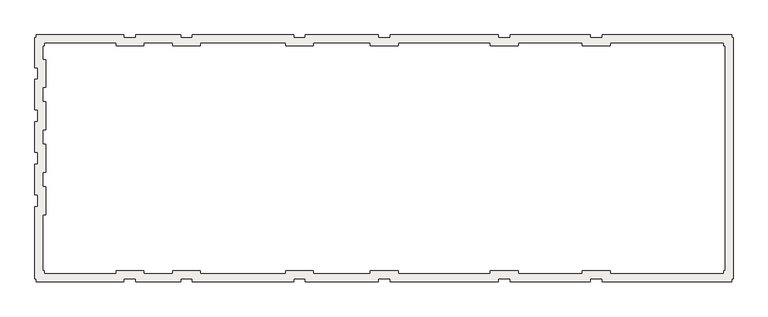
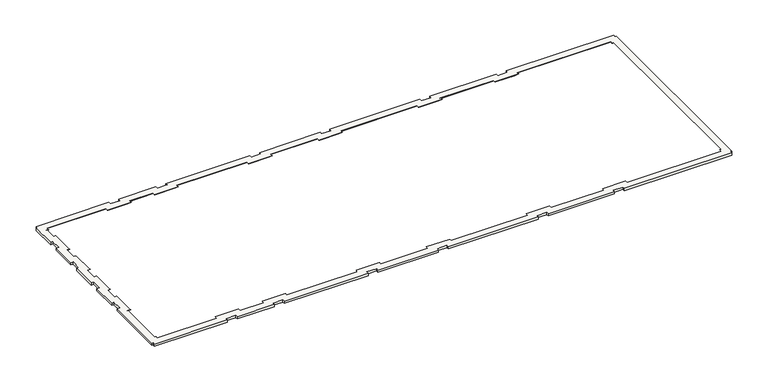
"""IFC4 building model written with IfcOpenShell, lengths in millimetres: slab geometry, HAUNCH FOR SOG : FTS801_Haunch_GS."""

import ifcopenshell
import ifcopenshell.guid

model = None  # the IFC model being written
_history = None  # IfcOwnerHistory: only IFC2X3 demands one
_inside = {}  # id of a spatial element -> (the spatial element, [elements in it])
_under = {}  # id of a project, library or spatial element -> (it, [spatial elements below it])
_declared = {}  # id of a project -> (the project, [libraries it declares])
_typed = {}  # id of a type object -> (the type object, [elements of that type])
_made_of = {}  # id of a material, layer set ... -> (it, [elements and type objects made of it])


def new_model(schema):
    """Start an empty IFC model of exactly this schema.

    Asked for "IFC4X3", IfcOpenShell would pick the latest addendum, in which some entities
    have other attributes; the version numbers below select the first issue.
    IFC2X3 requires an IfcOwnerHistory on every rooted entity: one is made here for all.
    """
    global model, _history
    if schema == "IFC4X3":
        model = ifcopenshell.file(schema_version=(4, 3, 0, 0))
    else:
        model = ifcopenshell.file(schema=schema)
    _inside.clear()
    _under.clear()
    _declared.clear()
    _typed.clear()
    _made_of.clear()
    _history = None
    if model.schema == "IFC2X3":
        org = make("IfcOrganization", Name="unknown")
        user = make(
            "IfcPersonAndOrganization",
            ThePerson=make("IfcPerson", FamilyName="unknown"),
            TheOrganization=org,
        )
        app = make(
            "IfcApplication",
            ApplicationDeveloper=org,
            Version="unknown",
            ApplicationFullName="unknown",
            ApplicationIdentifier="unknown",
        )
        _history = make(
            "IfcOwnerHistory",
            OwningUser=user,
            OwningApplication=app,
            ChangeAction="ADDED",
            CreationDate=0,
        )
    return model


def make(cls, **values):
    """One entity of the class cls with the attributes given. An attribute that is None is left unset."""
    return model.create_entity(
        cls, **{name: value for name, value in values.items() if value is not None}
    )


def rooted(cls, **values):
    """An entity with a GlobalId (a new one), such as an element, a storey or a relation."""
    return make(cls, GlobalId=ifcopenshell.guid.new(), OwnerHistory=_history, **values)


def si_unit(unit_type, name, prefix=None):
    """IfcSIUnit, for example si_unit("LENGTHUNIT", "METRE", prefix="MILLI")."""
    return make("IfcSIUnit", UnitType=unit_type, Prefix=prefix, Name=name)


def assignment(units):
    """IfcUnitAssignment: the units of a project."""
    return None if units is None else make("IfcUnitAssignment", Units=units)


def point(xyz):
    """IfcCartesianPoint."""
    return None if xyz is None else make("IfcCartesianPoint", Coordinates=xyz)


def direction(xyz):
    """IfcDirection."""
    return None if xyz is None else make("IfcDirection", DirectionRatios=xyz)


def frame(location, z_axis=None, x_axis=None):
    """IfcAxis2Placement3D, a coordinate frame: its origin and axes. An axis left out is left unset."""
    return make(
        "IfcAxis2Placement3D",
        Location=point(location),
        Axis=direction(z_axis),
        RefDirection=direction(x_axis),
    )


def origin():
    """The frame at (0, 0, 0) with its axes left unset."""
    return frame((0.0, 0.0, 0.0))


def place(relative_to, where):
    """IfcLocalPlacement: puts the frame where relative to a parent placement (None: the world)."""
    return make(
        "IfcLocalPlacement", PlacementRelTo=relative_to, RelativePlacement=where
    )


def context(
    kind, dimensions, precision=None, world=None, true_north=None, identifier=None
):
    """IfcGeometricRepresentationContext, for example the 3D "Model" context."""
    return make(
        "IfcGeometricRepresentationContext",
        ContextIdentifier=identifier,
        ContextType=kind,
        CoordinateSpaceDimension=dimensions,
        Precision=precision,
        WorldCoordinateSystem=world,
        TrueNorth=true_north,
    )


def project(units=None, contexts=None):
    """IfcProject with its units and contexts."""
    return rooted(
        "IfcProject",
        Name="project",
        RepresentationContexts=contexts,
        UnitsInContext=assignment(units),
    )


def spatial(cls, under=None, at=None, **own):
    """A site, building, storey or space (cls), placed at a placement, below another one or the project."""
    s = rooted(cls, ObjectPlacement=at, **own)
    if under is not None:
        _under.setdefault(under.id(), (under, []))[1].append(s)
    return s


def faces_of(points, faces, orient=None, outer=None):
    """IfcFace entities. A face is a list of loops; a loop is a list of indices into points, from 0.

    orient and outer hold one flag for each loop. By default every Orientation is true, the
    first loop of a face is its IfcFaceOuterBound and the others are IfcFaceBound.
    """
    made = []
    for i, loops in enumerate(faces):
        bounds = []
        for j, loop in enumerate(loops):
            is_outer = j == 0 if outer is None else outer[i][j]
            bounds.append(
                make(
                    "IfcFaceOuterBound" if is_outer else "IfcFaceBound",
                    Bound=make("IfcPolyLoop", Polygon=[points[k] for k in loop]),
                    Orientation=True if orient is None else orient[i][j],
                )
            )
        made.append(make("IfcFace", Bounds=bounds))
    return made


def faceted_brep(points, faces, orient=None, outer=None, voids=None):
    """IfcFacetedBrep: a solid bounded by flat faces; with voids (closed shells), ...WithVoids."""
    shared = [point(p) for p in points]
    hull = make("IfcClosedShell", CfsFaces=faces_of(shared, faces, orient, outer))
    if voids is None:
        return make("IfcFacetedBrep", Outer=hull)
    return make(
        "IfcFacetedBrepWithVoids",
        Outer=hull,
        Voids=[
            make(cls, CfsFaces=faces_of(shared, fs, o, b)) for cls, fs, o, b in voids
        ],
    )


def shape(context_of_items, identifier, shape_type, items):
    """IfcShapeRepresentation: the items that make up one representation, for example the "Body"."""
    return make(
        "IfcShapeRepresentation",
        ContextOfItems=context_of_items,
        RepresentationIdentifier=identifier,
        RepresentationType=shape_type,
        Items=items,
    )


def source(mapping_origin, context_of_items, identifier, shape_type, items):
    """IfcRepresentationMap: a shape defined once, which mapped items show again and again."""
    return make(
        "IfcRepresentationMap",
        MappingOrigin=mapping_origin,
        MappedRepresentation=shape(context_of_items, identifier, shape_type, items),
    )


def transform(
    local_origin,
    x_axis=None,
    y_axis=None,
    z_axis=None,
    scale=None,
    scale2=None,
    scale3=None,
    uniform=True,
):
    """IfcCartesianTransformationOperator3D, or its non-uniform kind. x_axis, y_axis, z_axis: its Axis1, 2, 3."""
    if uniform:
        return make(
            "IfcCartesianTransformationOperator3D",
            Axis1=direction(x_axis),
            Axis2=direction(y_axis),
            LocalOrigin=point(local_origin),
            Scale=scale,
            Axis3=direction(z_axis),
        )
    return make(
        "IfcCartesianTransformationOperator3DnonUniform",
        Axis1=direction(x_axis),
        Axis2=direction(y_axis),
        LocalOrigin=point(local_origin),
        Scale=scale,
        Axis3=direction(z_axis),
        Scale2=scale2,
        Scale3=scale3,
    )


def mapped(mapping_source, mapping_target):
    """IfcMappedItem: shows the shape of a source again, moved by a transform."""
    return make(
        "IfcMappedItem", MappingSource=mapping_source, MappingTarget=mapping_target
    )


def made_of(thing, what):
    """Note that an element or type object is made of a material, layer set ...; save() writes the relation."""
    if what is not None:
        _made_of.setdefault(what.id(), (what, []))[1].append(thing)
    return thing


def element(
    cls,
    number,
    at=None,
    inside=None,
    cuts=None,
    type_object=None,
    material=None,
    context=None,
    identifier="Body",
    shape_type=None,
    held_by="IfcProductDefinitionShape",
    body=None,
    shapes=None,
    **own,
):
    """One element of the class cls, such as IfcWall. Its Tag is "e" and its number.

    at: its placement. inside: the storey or other place that contains it. cuts: it is an
    opening in that element (IfcRelVoidsElement). A single representation is given by context,
    identifier, shape_type and body (its items); several are given by shapes. held_by: the class
    of the entity that holds the representations. save() writes the other relations.
    """
    e = rooted(cls, Tag="e%d" % number, ObjectPlacement=at, **own)
    if body is not None:
        shapes = [shape(context, identifier, shape_type, body)]
    if shapes is not None:
        e.Representation = make(held_by, Representations=shapes)
    if inside is not None:
        _inside.setdefault(inside.id(), (inside, []))[1].append(e)
    if cuts is not None:
        rooted(
            "IfcRelVoidsElement", RelatingBuildingElement=cuts, RelatedOpeningElement=e
        )
    if type_object is not None:
        _typed.setdefault(type_object.id(), (type_object, []))[1].append(e)
    return made_of(e, material)


def aggregate(whole, parts):
    """IfcRelAggregates: a whole, such as a stair, and the parts it consists of."""
    return rooted("IfcRelAggregates", RelatingObject=whole, RelatedObjects=parts)


def save(model, path):
    """Write the relations noted so far, then the file.

    IfcRelAggregates (storeys below a building ...), IfcRelContainedInSpatialStructure (elements
    in a storey), IfcRelDefinesByType, IfcRelAssociatesMaterial and IfcRelDeclares: one each for
    every whole, place, type object, material and project.
    """
    for whole, parts in _under.values():
        aggregate(whole, parts)
    for where, things in _inside.values():
        rooted(
            "IfcRelContainedInSpatialStructure",
            RelatedElements=things,
            RelatingStructure=where,
        )
    for kind, things in _typed.values():
        rooted("IfcRelDefinesByType", RelatedObjects=things, RelatingType=kind)
    for what, things in _made_of.values():
        rooted("IfcRelAssociatesMaterial", RelatedObjects=things, RelatingMaterial=what)
    for by, libraries in _declared.values():
        rooted("IfcRelDeclares", RelatingContext=by, RelatedDefinitions=libraries)
    model.write(path)


def slab_ae3d626d(model_context):
    return source(origin(), model_context, "Body", "Brep", [
        faceted_brep([(370.0, 38729.5208589, 399.9720055), (370.0, 38729.5208589, 199.9720055), (370.0, 38529.5208589, 199.9720055), (370.0, 38529.5208589, 399.9720055), (770.0, 38329.5208589, 199.9720055), (970.0, 38129.5208589, 399.9720055), (970.0, 37929.5208589, 399.9720055), (770.0, 38129.5208589, 199.9720055), (270.0, 38529.5208589, 199.9720055), (270.0, 38529.5208589, 399.9720055), (870.0, 37929.5208589, 399.9720055), (670.0, 38129.5208589, 199.9720055), (270.0, 36419.5208589, 199.9720055), (270.0, 36419.5208589, 399.9720055), (870.0, 37019.5208589, 399.9720055), (670.0, 36819.5208589, 199.9720055), (470.0, 36419.5208589, 199.9720055), (470.0, 36419.5208589, 399.9720055), (405.0, 36419.5208589, 399.9720055), (1070.0, 37019.5208589, 399.9720055), (870.0, 36819.5208589, 199.9720055), (470.0, 35579.5208589, 199.9720055), (470.0, 35579.5208589, 399.9720055), (1070.0, 34979.5208589, 399.9720055), (870.0, 35179.5208589, 199.9720055), (270.0, 35579.5208589, 199.9720055), (270.0, 35579.5208589, 399.9720055), (405.0, 35579.5208589, 399.9720055), (870.0, 34979.5208589, 399.9720055), (670.0, 35179.5208589, 199.9720055), (270.0, 33419.5208589, 199.9720055), (270.0, 33419.5208589, 399.9720055), (870.0, 34019.5208589, 399.9720055), (670.0, 33819.5208589, 199.9720055), (470.0, 33419.5208589, 199.9720055), (470.0, 33419.5208589, 399.9720055), (405.0, 33419.5208589, 399.9720055), (1070.0, 34019.5208589, 399.9720055), (870.0, 33819.5208589, 199.9720055), (470.0, 32579.5208589, 199.9720055), (470.0, 32579.5208589, 399.9720055), (1070.0, 31979.5208589, 399.9720055), (870.0, 32179.5208589, 199.9720055), (270.0, 32579.5208589, 199.9720055), (270.0, 32579.5208589, 399.9720055), (405.0, 32579.5208589, 399.9720055), (870.0, 31979.5208589, 399.9720055), (670.0, 32179.5208589, 199.9720055), (270.0, 30419.5208589, 199.9720055), (270.0, 30419.5208589, 399.9720055), (870.0, 31019.5208589, 399.9720055), (670.0, 30819.5208589, 199.9720055), (470.0, 30419.5208589, 199.9720055), (470.0, 30419.5208589, 399.9720055), (405.0, 30419.5208589, 399.9720055), (1070.0, 31019.5208589, 399.9720055), (870.0, 30819.5208589, 199.9720055), (470.0, 29579.5208589, 199.9720055), (470.0, 29579.5208589, 399.9720055), (1070.0, 28979.5208589, 399.9720055), (870.0, 29179.5208589, 199.9720055), (270.0, 29579.5208589, 199.9720055), (270.0, 29579.5208589, 399.9720055), (405.0, 29579.5208589, 399.9720055), (870.0, 28979.5208589, 399.9720055), (670.0, 29179.5208589, 199.9720055), (270.0, 27419.5208589, 199.9720055), (270.0, 27419.5208589, 399.9720055), (870.0, 28019.5208589, 399.9720055), (670.0, 27819.5208589, 199.9720055), (470.0, 27419.5208589, 199.9720055), (470.0, 27419.5208589, 399.9720055), (405.0, 27419.5208589, 399.9720055), (1070.0, 28019.5208589, 399.9720055), (870.0, 27819.5208589, 199.9720055), (470.0, 26579.5208589, 199.9720055), (470.0, 26579.5208589, 399.9720055), (1070.0, 25979.5208589, 399.9720055), (870.0, 26179.5208589, 199.9720055), (270.0, 26579.5208589, 199.9720055), (270.0, 26579.5208589, 399.9720055), (405.0, 26579.5208589, 399.9720055), (870.0, 25979.5208589, 399.9720055), (670.0, 26179.5208589, 199.9720055), (270.0, 21469.5208589, 199.9720055), (270.0, 21469.5208589, 399.9720055), (870.0, 22069.5208589, 399.9720055), (670.0, 21869.5208589, 199.9720055), (370.0, 21469.5208589, 199.9720055), (370.0, 21469.5208589, 399.9720055), (970.0, 22069.5208589, 399.9720055), (770.0, 21869.5208589, 199.9720055), (370.0, 21269.5208589, 199.9720055), (370.0, 21269.5208589, 399.9720055), (970.0, 21869.5208589, 399.9720055), (770.0, 21669.5208589, 199.9720055), (6574.0, 21269.5208589, 199.9720055), (6574.0, 21269.5208589, 399.9720055), (5974.0, 21869.5208589, 399.9720055), (6174.0, 21669.5208589, 199.9720055), (6574.0, 21469.5208589, 199.9720055), (6574.0, 21469.5208589, 399.9720055), (5974.0, 22069.5208589, 399.9720055), (6174.0, 21869.5208589, 199.9720055), (7414.0, 21469.5208589, 199.9720055), (7414.0, 21469.5208589, 399.9720055), (8014.0, 22069.5208589, 399.9720055), (7814.0, 21869.5208589, 199.9720055), (7414.0, 21269.5208589, 199.9720055), (7414.0, 21269.5208589, 399.9720055), (8014.0, 21869.5208589, 399.9720055), (7814.0, 21669.5208589, 199.9720055), (10574.0, 21269.5208589, 199.9720055), (10574.0, 21269.5208589, 399.9720055), (9974.0, 21869.5208589, 399.9720055), (10174.0, 21669.5208589, 199.9720055), (10574.0, 21469.5208589, 199.9720055), (10574.0, 21469.5208589, 399.9720055), (9974.0, 22069.5208589, 399.9720055), (10174.0, 21869.5208589, 199.9720055), (11414.0, 21469.5208589, 199.9720055), (11414.0, 21469.5208589, 399.9720055), (12014.0, 22069.5208589, 399.9720055), (11814.0, 21869.5208589, 199.9720055), (11414.0, 21269.5208589, 199.9720055), (11414.0, 21269.5208589, 399.9720055), (12014.0, 21869.5208589, 399.9720055), (11814.0, 21669.5208589, 199.9720055), (18574.0, 21269.5208589, 199.9720055), (18574.0, 21269.5208589, 399.9720055), (17974.0, 21869.5208589, 399.9720055), (18174.0, 21669.5208589, 199.9720055), (18574.0, 21469.5208589, 199.9720055), (18574.0, 21469.5208589, 399.9720055), (17974.0, 22069.5208589, 399.9720055), (18174.0, 21869.5208589, 199.9720055), (19414.0, 21469.5208589, 199.9720055), (19414.0, 21469.5208589, 399.9720055), (20014.0, 22069.5208589, 399.9720055), (19814.0, 21869.5208589, 199.9720055), (19414.0, 21269.5208589, 199.9720055), (19414.0, 21269.5208589, 399.9720055), (20014.0, 21869.5208589, 399.9720055), (19814.0, 21669.5208589, 199.9720055), (24574.0, 21269.5208589, 199.9720055), (24574.0, 21269.5208589, 399.9720055), (23974.0, 21869.5208589, 399.9720055), (24174.0, 21669.5208589, 199.9720055), (24574.0, 21469.5208589, 199.9720055), (24574.0, 21469.5208589, 399.9720055), (23974.0, 22069.5208589, 399.9720055), (24174.0, 21869.5208589, 199.9720055), (25414.0, 21469.5208589, 199.9720055), (25414.0, 21469.5208589, 399.9720055), (26014.0, 22069.5208589, 399.9720055), (25814.0, 21869.5208589, 199.9720055), (25414.0, 21269.5208589, 199.9720055), (25414.0, 21269.5208589, 399.9720055), (26014.0, 21869.5208589, 399.9720055), (25814.0, 21669.5208589, 199.9720055), (33074.0, 21269.5208589, 199.9720055), (33074.0, 21269.5208589, 399.9720055), (32474.0, 21869.5208589, 399.9720055), (32674.0, 21669.5208589, 199.9720055), (33074.0, 21469.5208589, 199.9720055), (33074.0, 21469.5208589, 399.9720055), (32474.0, 22069.5208589, 399.9720055), (32674.0, 21869.5208589, 199.9720055), (33914.0, 21469.5208589, 199.9720055), (33914.0, 21469.5208589, 399.9720055), (34514.0, 22069.5208589, 399.9720055), (34314.0, 21869.5208589, 199.9720055), (33914.0, 21269.5208589, 199.9720055), (33914.0, 21269.5208589, 399.9720055), (34514.0, 21869.5208589, 399.9720055), (34314.0, 21669.5208589, 199.9720055), (39574.0, 21269.5208589, 199.9720055), (39574.0, 21269.5208589, 399.9720055), (38974.0, 21869.5208589, 399.9720055), (39174.0, 21669.5208589, 199.9720055), (39574.0, 21469.5208589, 199.9720055), (39574.0, 21469.5208589, 399.9720055), (38974.0, 22069.5208589, 399.9720055), (39174.0, 21869.5208589, 199.9720055), (40414.0, 21469.5208589, 199.9720055), (40414.0, 21469.5208589, 399.9720055), (41014.0, 22069.5208589, 399.9720055), (40814.0, 21869.5208589, 199.9720055), (40414.0, 21269.5208589, 199.9720055), (40414.0, 21269.5208589, 399.9720055), (41014.0, 21869.5208589, 399.9720055), (40814.0, 21669.5208589, 199.9720055), (49580.0, 21269.5208589, 199.9720055), (49580.0, 21269.5208589, 399.9720055), (48980.0, 21869.5208589, 399.9720055), (49180.0, 21669.5208589, 199.9720055), (49580.0, 21469.5208589, 199.9720055), (49580.0, 21469.5208589, 399.9720055), (48980.0, 22069.5208589, 399.9720055), (49180.0, 21869.5208589, 199.9720055), (49680.0, 21469.5208589, 199.9720055), (49680.0, 21469.5208589, 399.9720055), (49595.0, 21469.5208589, 399.9720055), (49080.0, 22069.5208589, 399.9720055), (49280.0, 21869.5208589, 199.9720055), (49680.0, 38529.5208589, 199.9720055), (49680.0, 38529.5208589, 399.9720055), (49080.0, 37929.5208589, 399.9720055), (49280.0, 38129.5208589, 199.9720055), (49580.0, 38529.5208589, 199.9720055), (49580.0, 38529.5208589, 399.9720055), (49595.0, 38529.5208589, 399.9720055), (48980.0, 37929.5208589, 399.9720055), (49180.0, 38129.5208589, 199.9720055), (49580.0, 38729.5208589, 199.9720055), (49580.0, 38729.5208589, 399.9720055), (48980.0, 38129.5208589, 399.9720055), (49180.0, 38329.5208589, 199.9720055), (40414.0, 38729.5208589, 199.9720055), (40414.0, 38729.5208589, 399.9720055), (41014.0, 38129.5208589, 399.9720055), (40814.0, 38329.5208589, 199.9720055), (40414.0, 38529.5208589, 199.9720055), (40414.0, 38529.5208589, 399.9720055), (41014.0, 37929.5208589, 399.9720055), (40814.0, 38129.5208589, 199.9720055), (39574.0, 38529.5208589, 199.9720055), (39574.0, 38529.5208589, 399.9720055), (38974.0, 37929.5208589, 399.9720055), (39174.0, 38129.5208589, 199.9720055), (39574.0, 38729.5208589, 199.9720055), (39574.0, 38729.5208589, 399.9720055), (38974.0, 38129.5208589, 399.9720055), (39174.0, 38329.5208589, 199.9720055), (33914.0, 38729.5208589, 199.9720055), (33914.0, 38729.5208589, 399.9720055), (34514.0, 38129.5208589, 399.9720055), (34314.0, 38329.5208589, 199.9720055), (33914.0, 38529.5208589, 199.9720055), (33914.0, 38529.5208589, 399.9720055), (34514.0, 37929.5208589, 399.9720055), (34314.0, 38129.5208589, 199.9720055), (33074.0, 38529.5208589, 199.9720055), (33074.0, 38529.5208589, 399.9720055), (32474.0, 37929.5208589, 399.9720055), (32674.0, 38129.5208589, 199.9720055), (33074.0, 38729.5208589, 199.9720055), (33074.0, 38729.5208589, 399.9720055), (32474.0, 38129.5208589, 399.9720055), (32674.0, 38329.5208589, 199.9720055), (25414.0, 38729.5208589, 199.9720055), (25414.0, 38729.5208589, 399.9720055), (26014.0, 38129.5208589, 399.9720055), (25814.0, 38329.5208589, 199.9720055), (25414.0, 38529.5208589, 199.9720055), (25414.0, 38529.5208589, 399.9720055), (26014.0, 37929.5208589, 399.9720055), (25814.0, 38129.5208589, 199.9720055), (24574.0, 38529.5208589, 199.9720055), (24574.0, 38529.5208589, 399.9720055), (23974.0, 37929.5208589, 399.9720055), (24174.0, 38129.5208589, 199.9720055), (24574.0, 38729.5208589, 199.9720055), (24574.0, 38729.5208589, 399.9720055), (23974.0, 38129.5208589, 399.9720055), (24174.0, 38329.5208589, 199.9720055), (19414.0, 38729.5208589, 199.9720055), (19414.0, 38729.5208589, 399.9720055), (20014.0, 38129.5208589, 399.9720055), (19814.0, 38329.5208589, 199.9720055), (19414.0, 38529.5208589, 199.9720055), (19414.0, 38529.5208589, 399.9720055), (20014.0, 37929.5208589, 399.9720055), (19814.0, 38129.5208589, 199.9720055), (18574.0, 38529.5208589, 199.9720055), (18574.0, 38529.5208589, 399.9720055), (17974.0, 37929.5208589, 399.9720055), (18174.0, 38129.5208589, 199.9720055), (18574.0, 38729.5208589, 199.9720055), (18574.0, 38729.5208589, 399.9720055), (17974.0, 38129.5208589, 399.9720055), (18174.0, 38329.5208589, 199.9720055), (11414.0, 38729.5208589, 199.9720055), (11414.0, 38729.5208589, 399.9720055), (12014.0, 38129.5208589, 399.9720055), (11814.0, 38329.5208589, 199.9720055), (11414.0, 38529.5208589, 199.9720055), (11414.0, 38529.5208589, 399.9720055), (12014.0, 37929.5208589, 399.9720055), (11814.0, 38129.5208589, 199.9720055), (10574.0, 38529.5208589, 199.9720055), (10574.0, 38529.5208589, 399.9720055), (9974.0, 37929.5208589, 399.9720055), (10174.0, 38129.5208589, 199.9720055), (10574.0, 38729.5208589, 199.9720055), (10574.0, 38729.5208589, 399.9720055), (9974.0, 38129.5208589, 399.9720055), (10174.0, 38329.5208589, 199.9720055), (7414.0, 38729.5208589, 199.9720055), (7414.0, 38729.5208589, 399.9720055), (8014.0, 38129.5208589, 399.9720055), (7814.0, 38329.5208589, 199.9720055), (7414.0, 38529.5208589, 199.9720055), (7414.0, 38529.5208589, 399.9720055), (8014.0, 37929.5208589, 399.9720055), (7814.0, 38129.5208589, 199.9720055), (6574.0, 38529.5208589, 199.9720055), (6574.0, 38529.5208589, 399.9720055), (5974.0, 37929.5208589, 399.9720055), (6174.0, 38129.5208589, 199.9720055), (6574.0, 38729.5208589, 199.9720055), (6574.0, 38729.5208589, 399.9720055), (5974.0, 38129.5208589, 399.9720055), (6174.0, 38329.5208589, 199.9720055)], [[[0, 1, 2, 3]], [[4, 5, 6, 7]], [[3, 2, 8, 9]], [[7, 6, 10, 11]], [[9, 8, 12, 13]], [[11, 10, 14, 15]], [[13, 12, 16, 17, 18]], [[15, 14, 19, 20]], [[17, 16, 21, 22]], [[20, 19, 23, 24]], [[22, 21, 25, 26, 27]], [[24, 23, 28, 29]], [[26, 25, 30, 31]], [[29, 28, 32, 33]], [[31, 30, 34, 35, 36]], [[33, 32, 37, 38]], [[35, 34, 39, 40]], [[38, 37, 41, 42]], [[40, 39, 43, 44, 45]], [[42, 41, 46, 47]], [[44, 43, 48, 49]], [[47, 46, 50, 51]], [[49, 48, 52, 53, 54]], [[51, 50, 55, 56]], [[53, 52, 57, 58]], [[56, 55, 59, 60]], [[58, 57, 61, 62, 63]], [[60, 59, 64, 65]], [[62, 61, 66, 67]], [[65, 64, 68, 69]], [[67, 66, 70, 71, 72]], [[69, 68, 73, 74]], [[71, 70, 75, 76]], [[74, 73, 77, 78]], [[76, 75, 79, 80, 81]], [[78, 77, 82, 83]], [[80, 79, 84, 85]], [[83, 82, 86, 87]], [[85, 84, 88, 89]], [[87, 86, 90, 91]], [[89, 88, 92, 93]], [[91, 90, 94, 95]], [[93, 92, 96, 97]], [[95, 94, 98, 99]], [[97, 96, 100, 101]], [[99, 98, 102, 103]], [[101, 100, 104, 105]], [[103, 102, 106, 107]], [[105, 104, 108, 109]], [[107, 106, 110, 111]], [[109, 108, 112, 113]], [[111, 110, 114, 115]], [[113, 112, 116, 117]], [[115, 114, 118, 119]], [[117, 116, 120, 121]], [[119, 118, 122, 123]], [[121, 120, 124, 125]], [[123, 122, 126, 127]], [[125, 124, 128, 129]], [[127, 126, 130, 131]], [[129, 128, 132, 133]], [[131, 130, 134, 135]], [[133, 132, 136, 137]], [[135, 134, 138, 139]], [[137, 136, 140, 141]], [[139, 138, 142, 143]], [[141, 140, 144, 145]], [[143, 142, 146, 147]], [[145, 144, 148, 149]], [[147, 146, 150, 151]], [[149, 148, 152, 153]], [[151, 150, 154, 155]], [[153, 152, 156, 157]], [[155, 154, 158, 159]], [[157, 156, 160, 161]], [[159, 158, 162, 163]], [[161, 160, 164, 165]], [[163, 162, 166, 167]], [[165, 164, 168, 169]], [[167, 166, 170, 171]], [[169, 168, 172, 173]], [[171, 170, 174, 175]], [[173, 172, 176, 177]], [[175, 174, 178, 179]], [[177, 176, 180, 181]], [[179, 178, 182, 183]], [[181, 180, 184, 185]], [[183, 182, 186, 187]], [[185, 184, 188, 189]], [[187, 186, 190, 191]], [[189, 188, 192, 193]], [[191, 190, 194, 195]], [[193, 192, 196, 197]], [[195, 194, 198, 199]], [[197, 196, 200, 201, 202]], [[199, 198, 203, 204]], [[201, 200, 205, 206]], [[204, 203, 207, 208]], [[206, 205, 209, 210, 211]], [[208, 207, 212, 213]], [[210, 209, 214, 215]], [[213, 212, 216, 217]], [[215, 214, 218, 219]], [[217, 216, 220, 221]], [[219, 218, 222, 223]], [[221, 220, 224, 225]], [[223, 222, 226, 227]], [[225, 224, 228, 229]], [[227, 226, 230, 231]], [[229, 228, 232, 233]], [[231, 230, 234, 235]], [[233, 232, 236, 237]], [[235, 234, 238, 239]], [[237, 236, 240, 241]], [[239, 238, 242, 243]], [[241, 240, 244, 245]], [[243, 242, 246, 247]], [[245, 244, 248, 249]], [[247, 246, 250, 251]], [[249, 248, 252, 253]], [[251, 250, 254, 255]], [[253, 252, 256, 257]], [[255, 254, 258, 259]], [[257, 256, 260, 261]], [[259, 258, 262, 263]], [[261, 260, 264, 265]], [[263, 262, 266, 267]], [[265, 264, 268, 269]], [[267, 266, 270, 271]], [[269, 268, 272, 273]], [[271, 270, 274, 275]], [[273, 272, 276, 277]], [[275, 274, 278, 279]], [[277, 276, 280, 281]], [[279, 278, 282, 283]], [[281, 280, 284, 285]], [[283, 282, 286, 287]], [[285, 284, 288, 289]], [[287, 286, 290, 291]], [[289, 288, 292, 293]], [[291, 290, 294, 295]], [[293, 292, 296, 297]], [[295, 294, 298, 299]], [[297, 296, 300, 301]], [[299, 298, 302, 303]], [[301, 300, 304, 305]], [[303, 302, 306, 307]], [[305, 304, 308, 309]], [[307, 306, 310, 311]], [[309, 308, 312, 313]], [[311, 310, 1, 0]], [[303, 307, 311, 0, 3, 9, 13, 18, 17, 22, 27, 26, 31, 36, 35, 40, 45, 44, 49, 54, 53, 58, 63, 62, 67, 72, 71, 76, 81, 80, 85, 89, 93, 97, 101, 105, 109, 113, 117, 121, 125, 129, 133, 137, 141, 145, 149, 153, 157, 161, 165, 169, 173, 177, 181, 185, 189, 193, 197, 202, 201, 206, 211, 210, 215, 219, 223, 227, 231, 235, 239, 243, 247, 251, 255, 259, 263, 267, 271, 275, 279, 283, 287, 291, 295, 299], [5, 312, 308, 304, 300, 296, 292, 288, 284, 280, 276, 272, 268, 264, 260, 256, 252, 248, 244, 240, 236, 232, 228, 224, 220, 216, 212, 207, 203, 198, 194, 190, 186, 182, 178, 174, 170, 166, 162, 158, 154, 150, 146, 142, 138, 134, 130, 126, 122, 118, 114, 110, 106, 102, 98, 94, 90, 86, 82, 77, 73, 68, 64, 59, 55, 50, 46, 41, 37, 32, 28, 23, 19, 14, 10, 6]], [[313, 312, 5, 4]], [[1, 310, 306, 302, 298, 294, 290, 286, 282, 278, 274, 270, 266, 262, 258, 254, 250, 246, 242, 238, 234, 230, 226, 222, 218, 214, 209, 205, 200, 196, 192, 188, 184, 180, 176, 172, 168, 164, 160, 156, 152, 148, 144, 140, 136, 132, 128, 124, 120, 116, 112, 108, 104, 100, 96, 92, 88, 84, 79, 75, 70, 66, 61, 57, 52, 48, 43, 39, 34, 30, 25, 21, 16, 12, 8, 2], [305, 309, 313, 4, 7, 11, 15, 20, 24, 29, 33, 38, 42, 47, 51, 56, 60, 65, 69, 74, 78, 83, 87, 91, 95, 99, 103, 107, 111, 115, 119, 123, 127, 131, 135, 139, 143, 147, 151, 155, 159, 163, 167, 171, 175, 179, 183, 187, 191, 195, 199, 204, 208, 213, 217, 221, 225, 229, 233, 237, 241, 245, 249, 253, 257, 261, 265, 269, 273, 277, 281, 285, 289, 293, 297, 301]]]),
    ])


if __name__ == "__main__":
    model = new_model("IFC4")
    model_context = context("Model", 3, world=origin())
    ifc_project = project(units=[si_unit("LENGTHUNIT", "METRE", prefix="MILLI")], contexts=[model_context])
    site = spatial("IfcSite", under=ifc_project)
    building = spatial("IfcBuilding", under=site)
    placement = place(None, origin())
    slab_shape = slab_ae3d626d(model_context)
    element("IfcSlab", 1, ObjectType="HAUNCH FOR SOG : FTS801_Haunch_GS", at=placement, inside=building, context=model_context, shape_type="MappedRepresentation", body=[
        mapped(slab_shape, transform((0.0, 0.0, 0.0), x_axis=(1.0, 0.0, 0.0), y_axis=(0.0, 1.0, 0.0), z_axis=(0.0, 0.0, 1.0))),
    ])
    save(model, "model.ifc")

# Revit data of these elements
# Element 1 (IfcSlab, "HAUNCH FOR SOG : FTS801_Haunch_GS")
#   Materials on its faces: "A03AD032-00010_Structural Concrete_UG_20-24MPa"
# Materials
#   "A03AD032-00010_Structural Concrete_UG_20-24MPa": class "Concrete", colour RGB 176 176 176, transparency 0, Keynote = "09910.A1", Description = "Substructure Concrete / Cement Type-1 / 24MPa", Cost = 0
